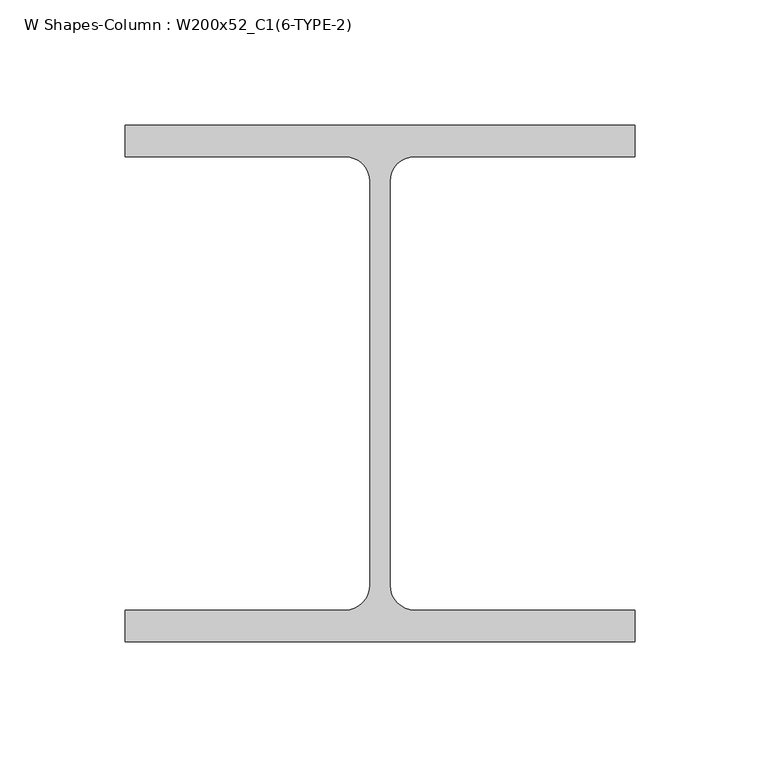
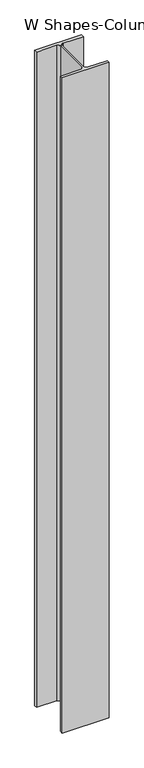
"""IFC4 building model written with IfcOpenShell, lengths in millimetres: column geometry, W Shapes-Column : W200x52_C1(6-TYPE-2)."""

from ifc_helpers import new_model, si_unit, point, frame, frame_2d, origin, place, context, project, spatial, polyline, circle_curve, trimmed, segment, composite_curve, outline, extrude, source, transform, mapped, element, save


def w_shapes_column_w200x52_c1_6_type_2_41c3fb3a(model_context):
    return source(origin(), model_context, "Body", "SweptSolid", [
        extrude(outline(composite_curve([segment(polyline([(101.854, -103.124), (-101.854, -103.124), (-101.854, -90.551), (-13.9446, -90.551)]), True, "CONTINUOUS"), segment(trimmed(circle_curve(frame_2d((-13.9446, -80.5434)), 10.0076), [point((-13.9446, -90.551))], [point((-3.937, -80.5434))], True, "CARTESIAN"), True, "CONTINUOUS"), segment(polyline([(-3.937, -80.5434), (-3.937, 80.5434)]), True, "CONTINUOUS"), segment(trimmed(circle_curve(frame_2d((-13.9446, 80.5434)), 10.0076), [point((-3.937, 80.5434))], [point((-13.9446, 90.551))], True, "CARTESIAN"), True, "CONTINUOUS"), segment(polyline([(-13.9446, 90.551), (-101.854, 90.551), (-101.854, 103.124), (101.854, 103.124), (101.854, 90.551), (13.9446, 90.551)]), True, "CONTINUOUS"), segment(trimmed(circle_curve(frame_2d((13.9446, 80.5434)), 10.0076), [point((13.9446, 90.551))], [point((3.937, 80.5434))], True, "CARTESIAN"), True, "CONTINUOUS"), segment(polyline([(3.937, 80.5434), (3.937, -80.5434)]), True, "CONTINUOUS"), segment(trimmed(circle_curve(frame_2d((13.9446, -80.5434)), 10.0076), [point((3.937, -80.5434))], [point((13.9446, -90.551))], True, "CARTESIAN"), True, "CONTINUOUS"), segment(polyline([(13.9446, -90.551), (101.854, -90.551), (101.854, -103.124)]), True, "CONTINUOUS")], self_intersect=False)), frame((0.0, 0.0, 200.0), z_axis=(0.0, 0.0, 1.0), x_axis=(1.0, 0.0, 0.0)), (0.0, 0.0, 1.0), 3000.0),
    ])


if __name__ == "__main__":
    model = new_model("IFC4")
    model_context = context("Model", 3, world=origin())
    ifc_project = project(units=[si_unit("LENGTHUNIT", "METRE", prefix="MILLI")], contexts=[model_context])
    site = spatial("IfcSite", under=ifc_project)
    building = spatial("IfcBuilding", under=site)
    placement = place(None, origin())
    w_shapes_column_w200x52_c1_6_type_2_shape = w_shapes_column_w200x52_c1_6_type_2_41c3fb3a(model_context)
    element("IfcColumn", 1, ObjectType="W Shapes-Column : W200x52_C1(6-TYPE-2)", at=placement, inside=building, context=model_context, shape_type="MappedRepresentation", body=[
        mapped(w_shapes_column_w200x52_c1_6_type_2_shape, transform((0.0, 0.0, 0.0), x_axis=(1.0, 0.0, 0.0), y_axis=(0.0, 1.0, 0.0), z_axis=(0.0, 0.0, 1.0))),
    ])
    save(model, "model.ifc")

# Revit data of these elements
# Type "W Shapes-Column : W200x52_C1(6-TYPE-2)"
#   Section Name Key = "W8X35"
#   Assembly Code = "B10"
#   Width = 20.3708 cm
#   Web Thickness = 0.7874 cm
#   Web Fillet = 1.0008 cm
#   Warping Constant = 166223.7 cm⁶
#   Torsional Moment of Inertia = 32.0082 cm⁴
#   Section Area = 66.4515 cm²
#   Plastic Modulus weak axis = 263.832 cm³
#   Plastic Modulus strong axis = 568.631 cm³
#   Perimeter = 1.1936 m²/m
#   Nominal Weight = 52.0857 kgf/m
#   Moment of Inertia weak axis = 1773.15 cm⁴
#   Moment of Inertia strong axis = 5286.14 cm⁴
#   Height = 20.6248 cm
#   Flange Thickness = 1.2573 cm
#   Elastic Modulus weak axis = 173.703 cm³
#   Elastic Modulus strong axis = 511.276 cm³
#   Clear Web Height = 14.605 cm
#   Centroid Vertical = 10.3124 cm
#   Centroid Horizontal = 10.1854 cm
#   Bolt Spacing = 13.97 cm
#   Structural Material [instance default] = Steel ASTM A992
#   Principal Axes Angle = 0
# Element 1 (IfcColumn, "W Shapes-Column : W200x52_C1(6-TYPE-2)")
#   Structural Material = none
# Materials
#   "Steel ASTM A992": class "Metal", colour RGB 199 199 199, transparency 0, Description = "Structural steel 50ksi", Cost = 0
